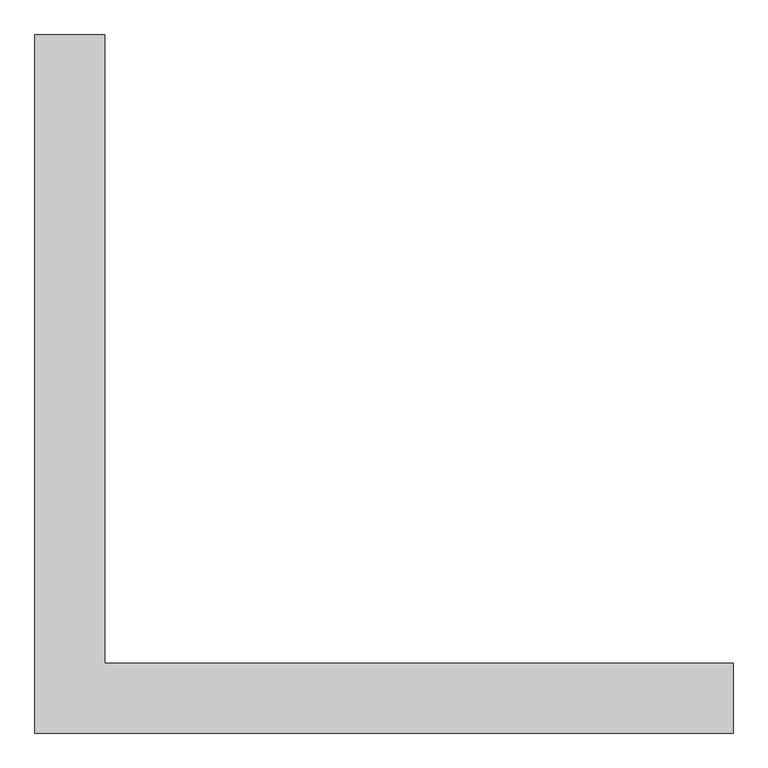
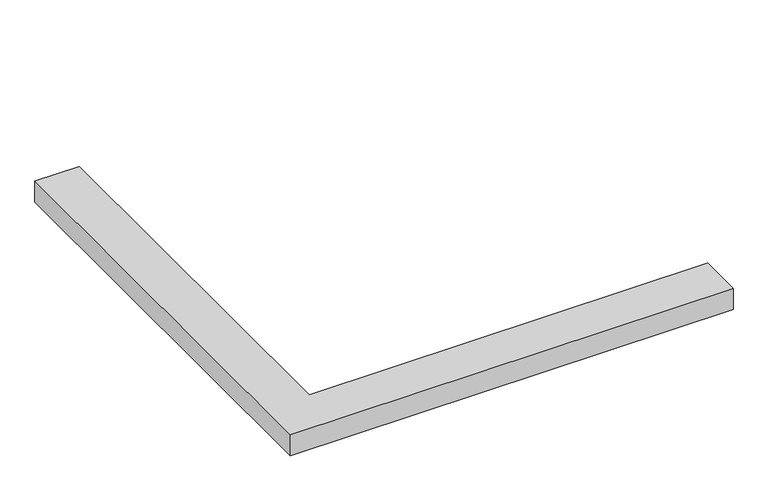
"""IFC4 building model written with IfcOpenShell, lengths in millimetres: proxy geometry, IN-EX_GM_NA_Origo : Origo."""

from ifc_helpers import new_model, si_unit, origin, origin_with_axes, place, context, project, spatial, polyline, outline, extrude, source, transform, mapped, element, save


def generic_models_3bfb9d1e(model_context):
    return source(origin(), model_context, "Body", "SweptSolid", [
        extrude(outline(polyline([(0.0, 0.0), (0.0, 1000.0), (100.0, 1000.0), (100.0, 100.0), (1000.0, 100.0), (1000.0, 0.0), (0.0, 0.0)])), origin_with_axes(), (0.0, 0.0, 1.0), 50.0),
    ])


if __name__ == "__main__":
    model = new_model("IFC4")
    model_context = context("Model", 3, world=origin())
    ifc_project = project(units=[si_unit("LENGTHUNIT", "METRE", prefix="MILLI")], contexts=[model_context])
    site = spatial("IfcSite", under=ifc_project)
    building = spatial("IfcBuilding", under=site)
    placement = place(None, origin())
    generic_models_shape = generic_models_3bfb9d1e(model_context)
    element("IfcBuildingElementProxy", 1, Name="IN-EX_GM_NA_Origo : Origo", ObjectType="IN-EX_GM_NA_Origo : Origo", at=placement, inside=building, context=model_context, shape_type="MappedRepresentation", body=[
        mapped(generic_models_shape, transform((0.0, 0.0, 0.0), x_axis=(1.0, 0.0, 0.0), y_axis=(0.0, 1.0, 0.0), z_axis=(0.0, 0.0, 1.0))),
    ])
    save(model, "model.ifc")

# Revit data of these elements
# Project information
#   ModelCreatedBy = "STUDIO IN-EX"
#   RevitTemplateDate = "251122_0345"
#   RevitVersion = "2026.3 - 26.3.0.37"
#   Building Code = "Building Code"
#   Organization Name = "STUDIO IN-EX Zrt."
#   Organization Description = "Architects & Engineers"
#   Building Name = "Building Name"
#   Author = "Structural"
#   ModelReference = "File Name"
#   Project Issue Date = "Issue Date"
#   Project Status = "Project  Status"
#   Client Name = "Client"
#   Project Address = "Project Address"
#   Project Name = "Project Name"
#   Project Number = "Main Project Code"
#   SR Document GUID = "2968e9a8-c7f4-4164-9e0d-14a0b04d7404"
#   Land Parcel = "Parcel Nr."
#   MC Version Saved = "2022.0"
# Type "IN-EX_GM_NA_Origo : Origo"
#   Copyright = "Copyright © 2019 Studio IN-EX Zrt. All rights reserved."
#   Assembly Code = "Z0000"
#   Default Elevation = 0
